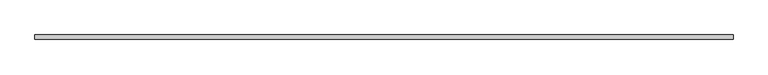
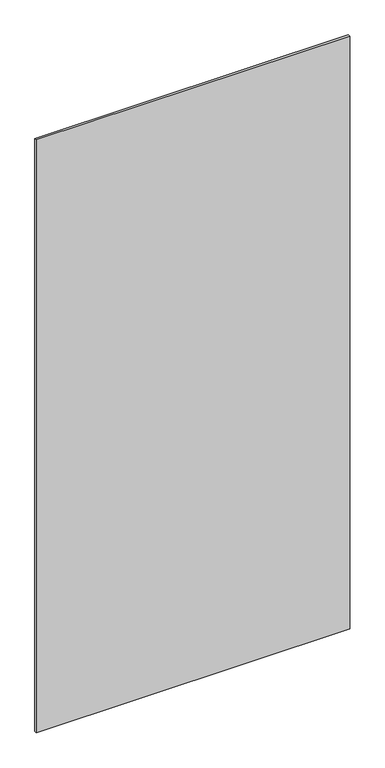
"""IFC4 building model written with IfcOpenShell, lengths in millimetres: proxy geometry, Panel:Panel:300402:Panel:300402 : Panel:Panel:300402:300124:Panel:300402:Panel:300402 : Panel:Panel:300402:300124 : Panel:Panel:300402:Panel:300402 : Panel:Panel:300402:300124:11 : Panel:Panel:300402:Panel:300402 : Panel:Panel:300402:300124:Panel:300402:Panel:300402 : Panel:Panel:300402:300124 : Panel:Panel:300402:Panel:300402 : Panel:Panel:300402:300124:300083."""

import ifcopenshell
import ifcopenshell.guid

model = None  # the IFC model being written
_history = None  # IfcOwnerHistory: only IFC2X3 demands one
_inside = {}  # id of a spatial element -> (the spatial element, [elements in it])
_under = {}  # id of a project, library or spatial element -> (it, [spatial elements below it])
_declared = {}  # id of a project -> (the project, [libraries it declares])
_typed = {}  # id of a type object -> (the type object, [elements of that type])
_made_of = {}  # id of a material, layer set ... -> (it, [elements and type objects made of it])


def new_model(schema):
    """Start an empty IFC model of exactly this schema.

    Asked for "IFC4X3", IfcOpenShell would pick the latest addendum, in which some entities
    have other attributes; the version numbers below select the first issue.
    IFC2X3 requires an IfcOwnerHistory on every rooted entity: one is made here for all.
    """
    global model, _history
    if schema == "IFC4X3":
        model = ifcopenshell.file(schema_version=(4, 3, 0, 0))
    else:
        model = ifcopenshell.file(schema=schema)
    _inside.clear()
    _under.clear()
    _declared.clear()
    _typed.clear()
    _made_of.clear()
    _history = None
    if model.schema == "IFC2X3":
        org = make("IfcOrganization", Name="unknown")
        user = make(
            "IfcPersonAndOrganization",
            ThePerson=make("IfcPerson", FamilyName="unknown"),
            TheOrganization=org,
        )
        app = make(
            "IfcApplication",
            ApplicationDeveloper=org,
            Version="unknown",
            ApplicationFullName="unknown",
            ApplicationIdentifier="unknown",
        )
        _history = make(
            "IfcOwnerHistory",
            OwningUser=user,
            OwningApplication=app,
            ChangeAction="ADDED",
            CreationDate=0,
        )
    return model


def make(cls, **values):
    """One entity of the class cls with the attributes given. An attribute that is None is left unset."""
    return model.create_entity(
        cls, **{name: value for name, value in values.items() if value is not None}
    )


def rooted(cls, **values):
    """An entity with a GlobalId (a new one), such as an element, a storey or a relation."""
    return make(cls, GlobalId=ifcopenshell.guid.new(), OwnerHistory=_history, **values)


def si_unit(unit_type, name, prefix=None):
    """IfcSIUnit, for example si_unit("LENGTHUNIT", "METRE", prefix="MILLI")."""
    return make("IfcSIUnit", UnitType=unit_type, Prefix=prefix, Name=name)


def assignment(units):
    """IfcUnitAssignment: the units of a project."""
    return None if units is None else make("IfcUnitAssignment", Units=units)


def point(xyz):
    """IfcCartesianPoint."""
    return None if xyz is None else make("IfcCartesianPoint", Coordinates=xyz)


def direction(xyz):
    """IfcDirection."""
    return None if xyz is None else make("IfcDirection", DirectionRatios=xyz)


def frame(location, z_axis=None, x_axis=None):
    """IfcAxis2Placement3D, a coordinate frame: its origin and axes. An axis left out is left unset."""
    return make(
        "IfcAxis2Placement3D",
        Location=point(location),
        Axis=direction(z_axis),
        RefDirection=direction(x_axis),
    )


def origin():
    """The frame at (0, 0, 0) with its axes left unset."""
    return frame((0.0, 0.0, 0.0))


def place(relative_to, where):
    """IfcLocalPlacement: puts the frame where relative to a parent placement (None: the world)."""
    return make(
        "IfcLocalPlacement", PlacementRelTo=relative_to, RelativePlacement=where
    )


def context(
    kind, dimensions, precision=None, world=None, true_north=None, identifier=None
):
    """IfcGeometricRepresentationContext, for example the 3D "Model" context."""
    return make(
        "IfcGeometricRepresentationContext",
        ContextIdentifier=identifier,
        ContextType=kind,
        CoordinateSpaceDimension=dimensions,
        Precision=precision,
        WorldCoordinateSystem=world,
        TrueNorth=true_north,
    )


def project(units=None, contexts=None):
    """IfcProject with its units and contexts."""
    return rooted(
        "IfcProject",
        Name="project",
        RepresentationContexts=contexts,
        UnitsInContext=assignment(units),
    )


def spatial(cls, under=None, at=None, **own):
    """A site, building, storey or space (cls), placed at a placement, below another one or the project."""
    s = rooted(cls, ObjectPlacement=at, **own)
    if under is not None:
        _under.setdefault(under.id(), (under, []))[1].append(s)
    return s


def polyline(points):
    """IfcPolyline through the points."""
    return make("IfcPolyline", Points=[point(p) for p in points])


def outline(outer, holes=None, kind="AREA"):
    """IfcArbitraryClosedProfileDef: a profile drawn as a closed curve; with holes, ...WithVoids."""
    if holes is None:
        return make("IfcArbitraryClosedProfileDef", ProfileType=kind, OuterCurve=outer)
    return make(
        "IfcArbitraryProfileDefWithVoids",
        ProfileType=kind,
        OuterCurve=outer,
        InnerCurves=holes,
    )


def extrude(swept, where, along, depth):
    """IfcExtrudedAreaSolid: the profile swept, set in the frame where, extruded along a direction by depth."""
    return make(
        "IfcExtrudedAreaSolid",
        SweptArea=swept,
        Position=where,
        ExtrudedDirection=direction(along),
        Depth=depth,
    )


def shape(context_of_items, identifier, shape_type, items):
    """IfcShapeRepresentation: the items that make up one representation, for example the "Body"."""
    return make(
        "IfcShapeRepresentation",
        ContextOfItems=context_of_items,
        RepresentationIdentifier=identifier,
        RepresentationType=shape_type,
        Items=items,
    )


def source(mapping_origin, context_of_items, identifier, shape_type, items):
    """IfcRepresentationMap: a shape defined once, which mapped items show again and again."""
    return make(
        "IfcRepresentationMap",
        MappingOrigin=mapping_origin,
        MappedRepresentation=shape(context_of_items, identifier, shape_type, items),
    )


def transform(
    local_origin,
    x_axis=None,
    y_axis=None,
    z_axis=None,
    scale=None,
    scale2=None,
    scale3=None,
    uniform=True,
):
    """IfcCartesianTransformationOperator3D, or its non-uniform kind. x_axis, y_axis, z_axis: its Axis1, 2, 3."""
    if uniform:
        return make(
            "IfcCartesianTransformationOperator3D",
            Axis1=direction(x_axis),
            Axis2=direction(y_axis),
            LocalOrigin=point(local_origin),
            Scale=scale,
            Axis3=direction(z_axis),
        )
    return make(
        "IfcCartesianTransformationOperator3DnonUniform",
        Axis1=direction(x_axis),
        Axis2=direction(y_axis),
        LocalOrigin=point(local_origin),
        Scale=scale,
        Axis3=direction(z_axis),
        Scale2=scale2,
        Scale3=scale3,
    )


def mapped(mapping_source, mapping_target):
    """IfcMappedItem: shows the shape of a source again, moved by a transform."""
    return make(
        "IfcMappedItem", MappingSource=mapping_source, MappingTarget=mapping_target
    )


def made_of(thing, what):
    """Note that an element or type object is made of a material, layer set ...; save() writes the relation."""
    if what is not None:
        _made_of.setdefault(what.id(), (what, []))[1].append(thing)
    return thing


def element(
    cls,
    number,
    at=None,
    inside=None,
    cuts=None,
    type_object=None,
    material=None,
    context=None,
    identifier="Body",
    shape_type=None,
    held_by="IfcProductDefinitionShape",
    body=None,
    shapes=None,
    **own,
):
    """One element of the class cls, such as IfcWall. Its Tag is "e" and its number.

    at: its placement. inside: the storey or other place that contains it. cuts: it is an
    opening in that element (IfcRelVoidsElement). A single representation is given by context,
    identifier, shape_type and body (its items); several are given by shapes. held_by: the class
    of the entity that holds the representations. save() writes the other relations.
    """
    e = rooted(cls, Tag="e%d" % number, ObjectPlacement=at, **own)
    if body is not None:
        shapes = [shape(context, identifier, shape_type, body)]
    if shapes is not None:
        e.Representation = make(held_by, Representations=shapes)
    if inside is not None:
        _inside.setdefault(inside.id(), (inside, []))[1].append(e)
    if cuts is not None:
        rooted(
            "IfcRelVoidsElement", RelatingBuildingElement=cuts, RelatedOpeningElement=e
        )
    if type_object is not None:
        _typed.setdefault(type_object.id(), (type_object, []))[1].append(e)
    return made_of(e, material)


def aggregate(whole, parts):
    """IfcRelAggregates: a whole, such as a stair, and the parts it consists of."""
    return rooted("IfcRelAggregates", RelatingObject=whole, RelatedObjects=parts)


def save(model, path):
    """Write the relations noted so far, then the file.

    IfcRelAggregates (storeys below a building ...), IfcRelContainedInSpatialStructure (elements
    in a storey), IfcRelDefinesByType, IfcRelAssociatesMaterial and IfcRelDeclares: one each for
    every whole, place, type object, material and project.
    """
    for whole, parts in _under.values():
        aggregate(whole, parts)
    for where, things in _inside.values():
        rooted(
            "IfcRelContainedInSpatialStructure",
            RelatedElements=things,
            RelatingStructure=where,
        )
    for kind, things in _typed.values():
        rooted("IfcRelDefinesByType", RelatedObjects=things, RelatingType=kind)
    for what, things in _made_of.values():
        rooted("IfcRelAssociatesMaterial", RelatedObjects=things, RelatingMaterial=what)
    for by, libraries in _declared.values():
        rooted("IfcRelDeclares", RelatingContext=by, RelatedDefinitions=libraries)
    model.write(path)


def generic_models_711a28cc(model_context):
    return source(origin(), model_context, "Body", "SweptSolid", [
        extrude(outline(polyline([(577805.9367239, -579076.8913841), (579025.1367239, -579076.8913841), (579025.1367239, -579084.8288841), (577805.9367239, -579084.8288841), (577805.9367239, -579076.8913841)])), frame((0.0, 0.0, 3695.7), z_axis=(0.0, 0.0, 1.0), x_axis=(1.0, 0.0, 0.0)), (0.0, 0.0, 1.0), 2438.4),
    ])


if __name__ == "__main__":
    model = new_model("IFC4")
    model_context = context("Model", 3, world=origin())
    ifc_project = project(units=[si_unit("LENGTHUNIT", "METRE", prefix="MILLI")], contexts=[model_context])
    site = spatial("IfcSite", under=ifc_project)
    building = spatial("IfcBuilding", under=site)
    placement = place(None, origin())
    generic_models_shape = generic_models_711a28cc(model_context)
    element("IfcBuildingElementProxy", 1, Name="Panel:Panel:300402:Panel:300402 : Panel:Panel:300402:300124:Panel:300402:Panel:300402 : Panel:Panel:300402:300124 : Panel:Panel:300402:Panel:300402 : Panel:Panel:300402:300124:11 : Panel:Panel:300402:Panel:300402 : Panel:Panel:300402:300124:Panel:300402:Panel:300402 : Panel:Panel:300402:300124 : Panel:Panel:300402:Panel:300402 : Panel:Panel:300402:300124:300083", ObjectType="Panel:Panel:300402:Panel:300402 : Panel:Panel:300402:300124:Panel:300402:Panel:300402 : Panel:Panel:300402:300124 : Panel:Panel:300402:Panel:300402 : Panel:Panel:300402:300124:11 : Panel:Panel:300402:Panel:300402 : Panel:Panel:300402:300124:Panel:300402:Panel:300402 : Panel:Panel:300402:300124 : Panel:Panel:300402:Panel:300402 : Panel:Panel:300402:300124:300083", at=placement, inside=building, context=model_context, shape_type="MappedRepresentation", body=[
        mapped(generic_models_shape, transform((0.0, 0.0, 0.0), x_axis=(1.0, 0.0, 0.0), y_axis=(0.0, 1.0, 0.0), z_axis=(0.0, 0.0, 1.0))),
    ])
    save(model, "model.ifc")

# Revit data of these elements
# Type "Panel:Panel:300402:Panel:300402 : Panel:Panel:300402:300124:Panel:300402:Panel:300402 : Panel:Panel:300402:300124 : Panel:Panel:300402:Panel:300402 : Panel:Panel:300402:300124:11 : Panel:Panel:300402:Panel:300402 : Panel:Panel:300402:300124:Panel:300402:Panel:300402 : Panel:Panel:300402:300124 : Panel:Panel:300402:Panel:300402 : Panel:Panel:300402:300124:300083"
#   NameOverride = "Panel:Panel:300402:Panel:300402 : Panel:Panel:300402:300124:Panel:300402:Panel:300402 : Panel:Panel:300402:300124 : Panel:Panel:300402:Panel:300402 : Panel:Panel:300402:300124:300083"
#   ObjectTypeOverride = "Panel:300402:Panel:300402 : Panel:Panel:300402:300124 : Panel:Panel:300402:Panel:300402 : Panel:Panel:300402:300124"
#   Reference = "Panel"
#   Tag = "300083"
# Element 1 (IfcBuildingElementProxy, "Panel:Panel:300402:Panel:300402 : Panel:Panel:300402:300124:Panel:300402:Panel:300402 : Panel:Panel:300402:300124 : Panel:Panel:300402:Panel:300402 : Panel:Panel:300402:300124:11 : Panel:Panel:300402:Panel:300402 : Panel:Panel:300402:300124:Panel:300402:Panel:300402 : Panel:Panel:300402:300124 : Panel:Panel:300402:Panel:300402 : Panel:Panel:300402:300124:300083")
#   Materials on its faces: "5/16\" THICK STONEWOOD RESIN PANELS - EXPOSED FASTENERS"
# Materials
#   "5/16\" THICK STONEWOOD RESIN PANELS - EXPOSED FASTENERS": class "Unassigned", colour RGB 64 64 64, transparency 0, Keynote = "M07420000.01", Cost = 0
